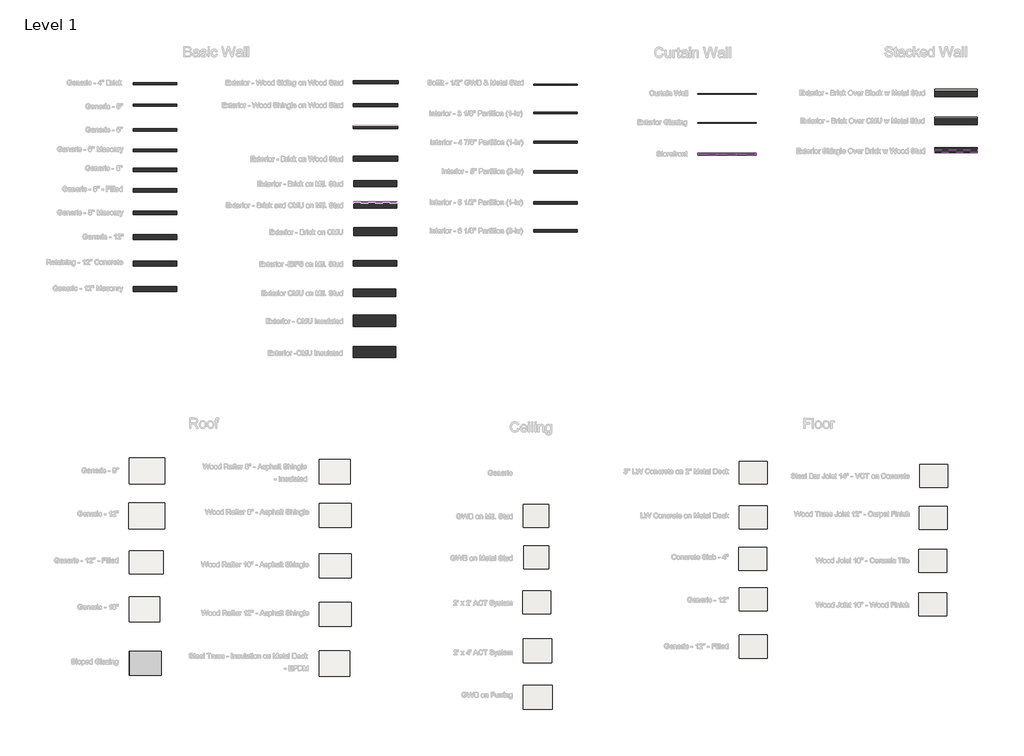
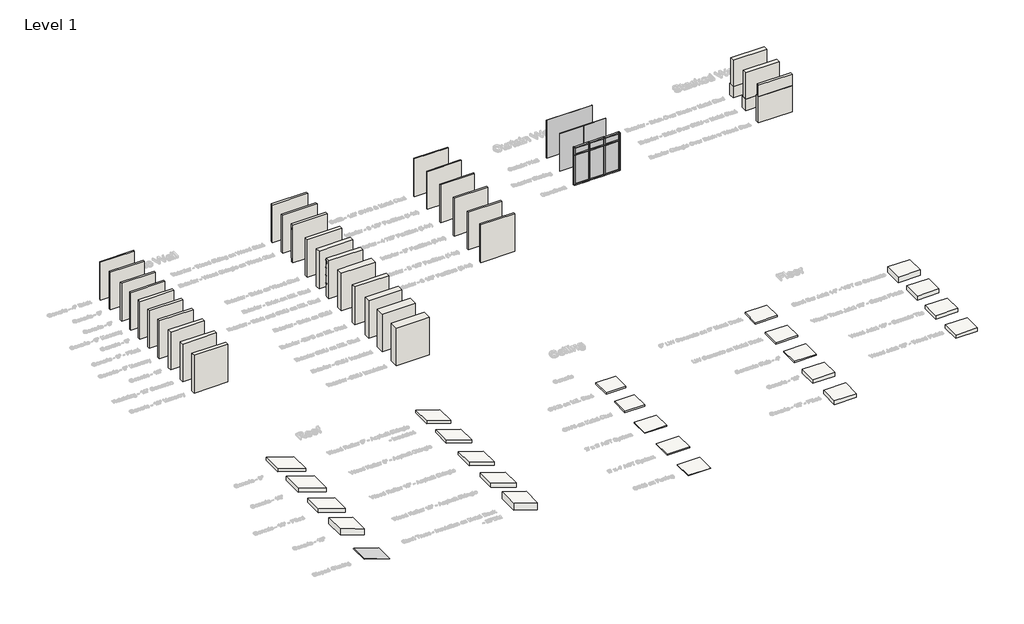
# One storey, part 1 of 42: 33 walls, 17 members, 10 plates, 9 roofs, 9 slabs, 5 coverings, 3 proxies.
# Revit data of these elements (continued)
# Type "Wood Joist 10\" - Wood Finish" (continued)
#   Layers, outside or top first: 0' - 0 3/4" "Oak Flooring" (function 4); 0' - 0 3/4" "Plywood, Sheathing" (function 1); 0' - 9 1/4" "Structure, Wood Joist/Rafter Layer" (function 1)
# Type "Soffit - 1/2\" GWB & Metal Stud"
#   Assembly Code = "B2010"
#   Layers, outside or top first: 0' - 1 1/2" "Metal Furring" (function 1); 0' - 0 1/2" "Gypsum Wall Board" (function 5)
# Type "Exterior - Wood Shingle over Wood Siding on Wood Stud"
#   Assembly Code = "B2010"
#   Layers, outside or top first: 0' - 0 5/8" "Wood Shake" (function 4); 0' - 0 5/8" "Siding, Clapboard" (function 4); 0' - 0" "Air Infiltration Barrier" (function 100); 0' - 0 3/4" "Plywood, Sheathing" (function 2); 0' - 5 1/2" "Softwood, Lumber" (function 1); 0' - 0" "Vapor Retarder" (function 100); 0' - 0 1/2" "Gypsum Wall Board" (function 5)
# Type "Exterior - Block on Mtl. Stud"
#   Layers, outside or top first: 0' - 7.87402" "Concrete Masonry Units" (function 4); 0' - 2.99213" "Air" (function 3); 0' - 0" "Air Infiltration Barrier" (function 100); 0' - 0.74803" "Plywood, Sheathing" (function 2); 0' - 5.98425" "Metal Stud Layer" (function 1); 0' - 0" "Vapour Retarder" (function 100); 0' - 0.51181" "Gypsum Wall Board" (function 5)
# Type "Exterior - Brick and CMU on MTL. Stud"
#   Assembly Code = "B2010"
#   Layers, outside or top first: 0' - 3 5/8" "Brick, Common" (function 4); 0' - 3 5/8" "Concrete Masonry Units" (function 4); 0' - 3" "Air" (function 3); 0' - 0" "Air Infiltration Barrier" (function 100); 0' - 0 3/4" "Plywood, Sheathing" (function 2); 0' - 6" "Metal Stud Layer" (function 1); 0' - 0" "Vapor Retarder" (function 100); 0' - 0 1/2" "Gypsum Wall Board" (function 5)
# Type "Exterior - Brick on CMU"
#   Assembly Code = "B2010156"
#   Layers, outside or top first: 0' - 3 5/8" "Brick, Common" (function 4); 0' - 3" "Air" (function 3); 0' - 3" "Rigid insulation" (function 3); 0' - 0" "Damp-proofing" (function 100); 0' - 7 5/8" "Concrete Masonry Units" (function 1); 0' - 1 5/8" "Metal Furring" (function 2); 0' - 0 5/8" "Gypsum Wall Board" (function 5)
# Type "Exterior - Brick on Mtl. Stud"
#   Assembly Code = "B2010158"
#   Layers, outside or top first: 0' - 3 5/8" "Brick, Common" (function 4); 0' - 3" "Air" (function 3); 0' - 0" "Air Infiltration Barrier" (function 100); 0' - 0 3/4" "Plywood, Sheathing" (function 2); 0' - 6" "Metal Stud Layer" (function 1); 0' - 0" "Vapor Retarder" (function 100); 0' - 0 1/2" "Gypsum Wall Board" (function 5)
# Type "Exterior - Brick on Wood Stud"
#   Assembly Code = "B2010158"
#   Layers, outside or top first: 0' - 3 5/8" "Brick, Common" (function 4); 0' - 1" "Air" (function 3); 0' - 0" "Air Infiltration Barrier" (function 100); 0' - 0 1/2" "Plywood, Sheathing" (function 2); 0' - 5 1/2" "Softwood, Lumber" (function 1); 0' - 0" "Vapor Retarder" (function 100); 0' - 0 1/2" "Gypsum Wall Board" (function 5)
# Type "Exterior - CMU Insulated"
#   Assembly Code = "B2010144"
#   Layers, outside or top first: 0' - 7 5/8" "Concrete Masonry Units" (function 1); 0' - 2" "Air" (function 3); 0' - 3" "Rigid insulation" (function 3); 0' - 0" "Damp-proofing" (function 100); 0' - 11 5/8" "Concrete Masonry Units" (function 1); 0' - 1 5/8" "Metal Furring" (function 2); 0' - 0 5/8" "Gypsum Wall Board" (function 5)
# Type "Exterior - CMU on Mtl. Stud"
#   Assembly Code = "B2010158"
#   Layers, outside or top first: 0' - 7 5/8" "Concrete Masonry Units" (function 4); 0' - 3" "Air" (function 3); 0' - 0" "Air Infiltration Barrier" (function 100); 0' - 0 3/4" "Plywood, Sheathing" (function 2); 0' - 6" "Metal Stud Layer" (function 1); 0' - 0" "Vapor Retarder" (function 100); 0' - 0 1/2" "Gypsum Wall Board" (function 5)
# Type "Exterior - EIFS on Mtl. Stud"
#   Assembly Code = "B2010100"
#   Layers, outside or top first: 0' - 3" "EIFS, Exterior Insulation" (function 4); 0' - 2" "Air" (function 3); 0' - 0" "Air Infiltration Barrier" (function 100); 0' - 0 3/4" "Plywood, Sheathing" (function 2); 0' - 6" "Metal Stud Layer" (function 1); 0' - 0" "Vapor Retarder" (function 100); 0' - 0 1/2" "Gypsum Wall Board" (function 5)
# Type "Exterior - Wood Shingle on Wood Stud"
#   Assembly Code = "B2010100"
#   Layers, outside or top first: 0' - 0 5/8" "Wood Shake" (function 4); 0' - 0" "Air Infiltration Barrier" (function 100); 0' - 0 1/2" "Plywood, Sheathing" (function 2); 0' - 5 1/2" "Softwood, Lumber" (function 1); 0' - 0" "Vapor Retarder" (function 100); 0' - 0 1/2" "Gypsum Wall Board" (function 5)
# Type "Exterior - Wood Siding on Wood Stud"
#   Assembly Code = "B2010100"
#   Layers, outside or top first: 0' - 0 3/4" "Siding, Clapboard" (function 4); 0' - 0" "Air Infiltration Barrier" (function 100); 0' - 0 1/2" "Plywood, Sheathing" (function 2); 0' - 5 1/2" "Softwood, Lumber" (function 1); 0' - 0" "Vapor Retarder" (function 100); 0' - 0 1/2" "Gypsum Wall Board" (function 5)
# Type "Generic - 12\""
#   Assembly Code = "B2010"
#   Layers, outside or top first: 1' - 0" no material (function 1)
# Type "Generic - 12\" Masonry"
#   Assembly Code = "B2010"
#   Layers, outside or top first: 0' - 11 5/8" "Concrete Masonry Units" (function 1)
# Type "Generic - 4\" Brick"
#   Assembly Code = "B2010"
#   Layers, outside or top first: 0' - 4" "Brick, Common" (function 1)
# Type "Generic - 5\""
#   Assembly Code = "B2010"
#   Layers, outside or top first: 0' - 5" no material (function 1)
# Type "Generic - 6\""
#   Assembly Code = "B2010"
#   Layers, outside or top first: 0' - 6" no material (function 1)
# Type "Generic - 6\" Masonry"
#   Assembly Code = "B2010"
#   Layers, outside or top first: 0' - 5 5/8" "Concrete Masonry Units" (function 1)
# Type "Generic - 8\""
#   Assembly Code = "B2010"
#   Layers, outside or top first: 0' - 8" no material (function 1)
# Type "Generic - 8\" - Filled"
#   Assembly Code = "B2010"
#   Layers, outside or top first: 0' - 8" no material (function 1)
# Type "Generic - 8\" Masonry"
#   Assembly Code = "B2010"
#   Layers, outside or top first: 0' - 7 5/8" "Concrete Masonry Units" (function 1)
# Type "Interior - 3 1/8\" Partition (1-hr)"
#   Assembly Code = "C1010145"
#   Layers, outside or top first: 0' - 0 1/2" "Gypsum Wall Board" (function 5); 0' - 0 1/4" "Gypsum Wall Board" (function 5); 0' - 1 5/8" "Metal Stud Layer" (function 1); 0' - 0 1/4" "Gypsum Wall Board" (function 5); 0' - 0 1/2" "Gypsum Wall Board" (function 5)
# Type "Interior - 4 7/8\" Partition (1-hr)"
#   Assembly Code = "C1010145"
#   Layers, outside or top first: 0' - 0 5/8" "Gypsum Wall Board" (function 5); 0' - 3 5/8" "Metal Stud Layer" (function 1); 0' - 0 5/8" "Gypsum Wall Board" (function 5)
# Type "Interior - 5 1/2\" Partition (1-hr)"
#   Assembly Code = "C1010145"
#   Layers, outside or top first: 0' - 0 5/8" "Gypsum Wall Board" (function 5); 0' - 3 5/8" "Metal Stud Layer" (function 1); 0' - 0 5/8" "Gypsum Wall Board" (function 5); 0' - 0 5/8" "Gypsum Wall Board" (function 5)
# Type "Interior - 5\" Partition (2-hr)"
#   Assembly Code = "C1010145"
#   Layers, outside or top first: 0' - 0 5/8" "Gypsum Wall Board" (function 5); 0' - 0 5/8" "Gypsum Wall Board" (function 5); 0' - 2 1/2" "Metal Stud Layer" (function 1); 0' - 0 5/8" "Gypsum Wall Board" (function 5); 0' - 0 5/8" "Gypsum Wall Board" (function 5)
# Type "Interior - 6 1/8\" Partition (2-hr)"
#   Assembly Code = "C1010145"
#   Layers, outside or top first: 0' - 0 5/8" "Gypsum Wall Board" (function 5); 0' - 0 5/8" "Gypsum Wall Board" (function 5); 0' - 3 5/8" "Metal Stud Layer" (function 1); 0' - 0 5/8" "Gypsum Wall Board" (function 5); 0' - 0 5/8" "Gypsum Wall Board" (function 5)
# Type "Retaining - 12\" Concrete"
#   Layers, outside or top first: 1' - 0" "Concrete, Cast-in-Place gray" (function 1)
# Element 4 (IfcCovering, "2' x 2' ACT System")
#   Height Offset From Level = 1' - 0"
#   Phase Created = New Construction
#   Materials on its faces: "Acoustic Ceiling Tile 24 x 24", "Default"
# Element 5 (IfcCovering, "2' x 4' ACT System")
#   Height Offset From Level = 1' - 0"
#   Phase Created = New Construction
#   Materials on its faces: "Acoustic Ceiling Tile 24 x 48", "Default"
# Element 6 (IfcCovering, "GWB on Furring")
#   Height Offset From Level = 1' - 0"
#   Phase Created = New Construction
#   Materials on its faces: "Gypsum Wall Board", "Metal Stud Layer"
# Element 7 (IfcCovering, "GWB on Metal Stud")
#   Height Offset From Level = 1' - 0"
#   Phase Created = New Construction
#   Materials on its faces: "Gypsum Wall Board", "Metal Stud Layer"
# Element 8 (IfcCovering, "GWB on Mtl. Stud")
#   Height Offset From Level = 1' - 0"
#   Phase Created = New Construction
#   Materials on its faces: "Gypsum Wall Board", "Metal Stud Layer"
# Elements 9, 10, 11, 12, 13, 14, 15, 16, 17, 18, 19, 20, 21, 22, 23, 24, 25 (IfcMember, "Rectangular Mullion : 2.5\" x 5\" rectangular")
#   Phase Created = New Construction
#   Materials on its faces: "Aluminum"
# Elements 26, 27, 28, 29, 30, 31, 32, 33, 34, 35 (IfcPlate, "System Panel : Glazed")
#   Phase Created = New Construction
#   Materials on its faces: "Glass"
# Element 36 (IfcRoof, "Generic - 12\"")
#   built-in parameter 1001705 = 3.40154 (stored number, unit not read)
#   built-in parameter 1001710 = 33615
#   Phase Created = New Construction
#   Materials on its faces: "Default Roof"
# Element 37 (IfcRoof, "Generic - 12\" - Filled")
#   built-in parameter 1001705 = 3.29103 (stored number, unit not read)
#   built-in parameter 1001710 = 33615
#   Phase Created = New Construction
#   Materials on its faces: "Default Roof"
# Element 38 (IfcRoof, "Generic - 18\"")
#   built-in parameter 1001705 = 3.60503 (stored number, unit not read)
#   built-in parameter 1001710 = 33615
#   Phase Created = New Construction
#   Materials on its faces: "Default Roof"
# Element 39 (IfcRoof, "Generic - 9\"")
#   built-in parameter 1001705 = 3.1239 (stored number, unit not read)
#   built-in parameter 1001710 = 33615
#   Phase Created = New Construction
#   Materials on its faces: "Default Roof"
# Element 40 (IfcRoof, "Steel Truss - Insulation on Metal Deck - EPDM")
#   built-in parameter 1001705 = 3.88858 (stored number, unit not read)
#   built-in parameter 1001710 = 33615
#   Phase Created = New Construction
#   Materials on its faces: "Structure, Steel Bar Joist Layer", "Roofing, EPDM Membrane"
# Element 41 (IfcRoof, "Wood Rafter 10\" - Asphalt Shingle")
#   built-in parameter 1001705 = 3.00948 (stored number, unit not read)
#   built-in parameter 1001710 = 33615
#   Phase Created = New Construction
#   Materials on its faces: "Structure, Wood Joist/Rafter Layer, Batt Insulation", "Asphalt Shingle"
# Element 42 (IfcRoof, "Wood Rafter 12\" - Asphalt Shingle")
#   built-in parameter 1001705 = 3.18516 (stored number, unit not read)
#   built-in parameter 1001710 = 33615
#   Phase Created = New Construction
#   Materials on its faces: "Structure, Wood Joist/Rafter Layer, Batt Insulation", "Asphalt Shingle"
# Element 43 (IfcRoof, "Wood Rafter 8\" - Asphalt Shingle")
#   built-in parameter 1001705 = 2.8338 (stored number, unit not read)
#   built-in parameter 1001710 = 33615
#   Phase Created = New Construction
#   Materials on its faces: "Structure, Wood Joist/Rafter Layer, Batt Insulation", "Asphalt Shingle"
# Element 44 (IfcRoof, "Wood Rafter 8\" - Asphalt Shingle - Insulated")
#   built-in parameter 1001705 = 2.75956 (stored number, unit not read)
#   built-in parameter 1001710 = 33615
#   Phase Created = New Construction
#   Materials on its faces: "Structure, Wood Joist/Rafter Layer, Batt Insulation", "Asphalt Shingle"
# Element 45 (IfcSlab, "Wood Truss  Joist 12\" - Carpet Finish ")
#   Height Offset From Level = 0' - 0"
#   Phase Created = New Construction
#   Materials on its faces: "Structure, Wood Joist/Rafter Layer", "Carpet (1)"
# Element 46 (IfcSlab, "3\" LW Concrete on 2\" Metal Deck")
#   Height Offset From Level = 0' - 0"
#   Phase Created = New Construction
#   Materials on its faces: "Metal Deck", "Concrete, Lightweight"
# Element 47 (IfcSlab, "Concrete Slab - 4\"")
#   Height Offset From Level = 0' - 0"
#   Phase Created = New Construction
#   Materials on its faces: "Concrete, Cast-in-Place gray"
# Element 48 (IfcSlab, "Generic - 12\"")
#   Height Offset From Level = 0' - 0"
#   Phase Created = New Construction
#   Materials on its faces: "Default Floor"
# Element 49 (IfcSlab, "Generic - 12\" - Filled")
#   Height Offset From Level = 0' - 0"
#   Phase Created = New Construction
#   Materials on its faces: "Default Floor"
# Element 50 (IfcSlab, "LW Concrete on Metal Deck")
#   Height Offset From Level = 0' - 0"
#   Phase Created = New Construction
#   Materials on its faces: "Metal Deck", "Concrete, Lightweight"
# Element 51 (IfcSlab, "Steel Bar Joist 14\" - VCT on Concrete")
#   Height Offset From Level = 0' - 0"
#   Phase Created = New Construction
#   Materials on its faces: "Structure, Steel Bar Joist Layer", "Vinyl Composition Tile"
# Element 52 (IfcSlab, "Wood Joist 10\" - Ceramic Tile")
#   Height Offset From Level = 0' - 0"
#   Phase Created = New Construction
#   Materials on its faces: "Structure, Wood Joist/Rafter Layer", "Tile, Mosaic, Gray"
# Element 53 (IfcSlab, "Wood Joist 10\" - Wood Finish")
#   Height Offset From Level = 0' - 0"
#   Phase Created = New Construction
#   Materials on its faces: "Structure, Wood Joist/Rafter Layer", "Oak Flooring"
# Element 54 (IfcWall, "Soffit - 1/2\" GWB & Metal Stud")
#   Top Offset = 0' - 0"
#   Base Offset = 0' - 0"
#   Unconnected Height = 10' - 0"
#   wall height = 10' - 0"
#   Phase Created = New Construction
#   Base Constraint = Level 1
#   Materials on its faces: "Default Wall", "Gypsum Wall Board", "Metal Furring"
# Element 55 (IfcWall, "Exterior - Wood Shingle over Wood Siding on Wood Stud")
#   Top Offset = 0' - 0"
#   Base Offset = 0' - 0"
#   Unconnected Height = 10' - 0"
#   wall height = 10' - 0"
#   Phase Created = New Construction
#   Base Constraint = Level 1
#   Materials on its faces: "Default Wall", "Gypsum Wall Board", "Siding, Clapboard"
# Element 56 (IfcWall, "Exterior - Block on Mtl. Stud")
#   Top Offset = 0' - 0"
#   Base Offset = 0' - 0"
#   Unconnected Height = 2' - 11.43307"
#   wall height = 2' - 11.43307"
#   Phase Created = New Construction
#   Base Constraint = Level 1
#   Materials on its faces: "Default Wall", "Gypsum Wall Board", "Concrete Masonry Units"
# Element 57 (IfcWall, "Exterior - Brick and CMU on MTL. Stud")
#   Top Offset = 0' - 0"
#   Base Offset = 0' - 0"
#   Unconnected Height = 10' - 0"
#   wall height = 10' - 0"
#   Phase Created = New Construction
#   Base Constraint = Level 1
#   Materials on its faces: "Brick, Common", "Default Wall", "Concrete Masonry Units", "Gypsum Wall Board"
# Element 58 (IfcWall, "Exterior - Brick on CMU")
#   Top Offset = 0' - 0"
#   Base Offset = 0' - 0"
#   Unconnected Height = 10' - 0"
#   wall height = 10' - 0"
#   Phase Created = New Construction
#   Base Constraint = Level 1
#   Materials on its faces: "Default Wall", "Gypsum Wall Board", "Brick, Common"
# Element 59 (IfcWall, "Exterior - Brick on Mtl. Stud")
#   Top Offset = 0' - 0"
#   Base Offset = 0' - 0"
#   Unconnected Height = 10' - 0"
#   wall height = 10' - 0"
#   Phase Created = New Construction
#   Base Constraint = Level 1
#   Materials on its faces: "Default Wall", "Gypsum Wall Board", "Brick, Common"
# Element 60 (IfcWall, "Exterior - Brick on Mtl. Stud")
#   built-in parameter 1001111 = 2' - 11.43307"
#   Top Offset = 0' - 0"
#   Base Offset = 2' - 11.43307"
#   Unconnected Height = 7' - 0.56693"
#   wall height = 7' - 0.56693"
#   Phase Created = New Construction
#   Base Constraint = Level 1
#   Materials on its faces: "Default Wall", "Gypsum Wall Board", "Brick, Common"
# Element 61 (IfcWall, "Exterior - Brick on Mtl. Stud")
#   built-in parameter 1001111 = 3' - 0"
#   Top Offset = 0' - 0"
#   Base Offset = 3' - 0"
#   Unconnected Height = 7' - 0"
#   wall height = 7' - 0"
#   Phase Created = New Construction
#   Base Constraint = Level 1
#   Materials on its faces: "Default Wall", "Gypsum Wall Board", "Brick, Common"
# Element 62 (IfcWall, "Exterior - Brick on Wood Stud")
#   Top Offset = 0' - 0"
#   Base Offset = 0' - 0"
#   Unconnected Height = 10' - 0"
#   wall height = 10' - 0"
#   Phase Created = New Construction
#   Base Constraint = Level 1
#   Materials on its faces: "Default Wall", "Gypsum Wall Board", "Brick, Common"
# Element 63 (IfcWall, "Exterior - Brick on Wood Stud")
#   Top Offset = 0' - 0"
#   Base Offset = 0' - 0"
#   Unconnected Height = 7' - 0"
#   wall height = 7' - 0"
#   Phase Created = New Construction
#   Base Constraint = Level 1
#   Materials on its faces: "Default Wall", "Gypsum Wall Board", "Brick, Common"
# Elements 64, 65 (IfcWall, "Exterior - CMU Insulated")
#   Top Offset = 0' - 0"
#   Base Offset = 0' - 0"
#   Unconnected Height = 10' - 0"
#   wall height = 10' - 0"
#   Phase Created = New Construction
#   Base Constraint = Level 1
#   Materials on its faces: "Default Wall", "Gypsum Wall Board", "Concrete Masonry Units"
# Element 66 (IfcWall, "Exterior - CMU on Mtl. Stud")
#   Top Offset = 0' - 0"
#   Base Offset = 0' - 0"
#   Unconnected Height = 10' - 0"
#   wall height = 10' - 0"
#   Phase Created = New Construction
#   Base Constraint = Level 1
#   Materials on its faces: "Default Wall", "Gypsum Wall Board", "Concrete Masonry Units"
# Element 67 (IfcWall, "Exterior - CMU on Mtl. Stud")
#   Top Offset = 0' - 0"
#   Base Offset = 0' - 0"
#   Unconnected Height = 3' - 0"
#   wall height = 3' - 0"
#   Phase Created = New Construction
#   Base Constraint = Level 1
#   Materials on its faces: "Default Wall", "Gypsum Wall Board", "Concrete Masonry Units"
# Element 68 (IfcWall, "Exterior - EIFS on Mtl. Stud")
#   Top Offset = 0' - 0"
#   Base Offset = 0' - 0"
#   Unconnected Height = 10' - 0"
#   wall height = 10' - 0"
#   Phase Created = New Construction
#   Base Constraint = Level 1
#   Materials on its faces: "Default Wall", "Gypsum Wall Board", "EIFS, Exterior Insulation"
# Element 69 (IfcWall, "Exterior - Wood Shingle on Wood Stud")
#   Top Offset = 0' - 0"
#   Base Offset = 0' - 0"
#   Unconnected Height = 10' - 0"
#   wall height = 10' - 0"
#   Phase Created = New Construction
#   Base Constraint = Level 1
#   Materials on its faces: "Default Wall", "Gypsum Wall Board", "Wood Shake"
# Element 70 (IfcWall, "Exterior - Wood Shingle on Wood Stud")
#   built-in parameter 1001111 = 7' - 0"
#   Top Offset = 0' - 0"
#   Base Offset = 7' - 0"
#   Unconnected Height = 3' - 0"
#   wall height = 3' - 0"
#   Phase Created = New Construction
#   Base Constraint = Level 1
#   Materials on its faces: "Default Wall", "Gypsum Wall Board", "Wood Shake"
# Element 71 (IfcWall, "Exterior - Wood Siding on Wood Stud")
#   Top Offset = 0' - 0"
#   Base Offset = 0' - 0"
#   Unconnected Height = 10' - 0"
#   wall height = 10' - 0"
#   Phase Created = New Construction
#   Base Constraint = Level 1
#   Materials on its faces: "Default Wall", "Gypsum Wall Board", "Siding, Clapboard"
# Element 72 (IfcWall, "Generic - 12\"")
#   Top Offset = 0' - 0"
#   Base Offset = 0' - 0"
#   Unconnected Height = 10' - 0"
#   wall height = 10' - 0"
#   Phase Created = New Construction
#   Base Constraint = Level 1
#   Materials on its faces: "Default Wall"
# Element 73 (IfcWall, "Generic - 12\" Masonry")
#   Top Offset = 0' - 0"
#   Base Offset = 0' - 0"
#   Unconnected Height = 10' - 0"
#   wall height = 10' - 0"
#   Phase Created = New Construction
#   Base Constraint = Level 1
#   Materials on its faces: "Concrete Masonry Units"
# Element 74 (IfcWall, "Generic - 4\" Brick")
#   Top Offset = 0' - 0"
#   Base Offset = 0' - 0"
#   Unconnected Height = 10' - 0"
#   wall height = 10' - 0"
#   Phase Created = New Construction
#   Base Constraint = Level 1
#   Materials on its faces: "Brick, Common"
# Element 75 (IfcWall, "Generic - 5\"")
#   Top Offset = 0' - 0"
#   Base Offset = 0' - 0"
#   Unconnected Height = 10' - 0"
#   wall height = 10' - 0"
#   Phase Created = New Construction
#   Base Constraint = Level 1
#   Materials on its faces: "Default Wall"
# Element 76 (IfcWall, "Generic - 6\"")
#   Top Offset = 0' - 0"
#   Base Offset = 0' - 0"
#   Unconnected Height = 10' - 0"
#   wall height = 10' - 0"
#   Phase Created = New Construction
#   Base Constraint = Level 1
#   Materials on its faces: "Default Wall"
# Element 77 (IfcWall, "Generic - 6\" Masonry")
#   Top Offset = 0' - 0"
#   Base Offset = 0' - 0"
#   Unconnected Height = 10' - 0"
#   wall height = 10' - 0"
#   Phase Created = New Construction
#   Base Constraint = Level 1
#   Materials on its faces: "Concrete Masonry Units"
# Element 78 (IfcWall, "Generic - 8\"")
#   Top Offset = 0' - 0"
#   Base Offset = 0' - 0"
#   Unconnected Height = 10' - 0"
#   wall height = 10' - 0"
#   Phase Created = New Construction
#   Base Constraint = Level 1
#   Materials on its faces: "Default Wall"
# Element 79 (IfcWall, "Generic - 8\" - Filled")
#   Top Offset = 0' - 0"
#   Base Offset = 0' - 0"
#   Unconnected Height = 10' - 0"
#   wall height = 10' - 0"
#   Phase Created = New Construction
#   Base Constraint = Level 1
#   Materials on its faces: "Default Wall"
# Element 80 (IfcWall, "Generic - 8\" Masonry")
#   Top Offset = 0' - 0"
#   Base Offset = 0' - 0"
#   Unconnected Height = 10' - 0"
#   wall height = 10' - 0"
#   Phase Created = New Construction
#   Base Constraint = Level 1
#   Materials on its faces: "Concrete Masonry Units"
# Element 81 (IfcWall, "Interior - 3 1/8\" Partition (1-hr)")
#   Top Offset = 0' - 0"
#   Base Offset = 0' - 0"
#   wall height = 10' - 0"
#   Phase Created = New Construction
#   Base Constraint = Level 1
#   Top Constraint = Level 2
#   Materials on its faces: "Default Wall", "Gypsum Wall Board"
# Element 82 (IfcWall, "Interior - 4 7/8\" Partition (1-hr)")
#   Top Offset = 0' - 0"
#   Base Offset = 0' - 0"
#   wall height = 10' - 0"
#   Phase Created = New Construction
#   Base Constraint = Level 1
#   Top Constraint = Level 2
#   Materials on its faces: "Default Wall", "Gypsum Wall Board"
# Element 83 (IfcWall, "Interior - 5 1/2\" Partition (1-hr)")
#   Top Offset = 0' - 0"
#   Base Offset = 0' - 0"
#   wall height = 10' - 0"
#   Phase Created = New Construction
#   Base Constraint = Level 1
#   Top Constraint = Level 2
#   Materials on its faces: "Default Wall", "Gypsum Wall Board"
# Element 84 (IfcWall, "Interior - 5\" Partition (2-hr)")
#   Top Offset = 0' - 0"
#   Base Offset = 0' - 0"
#   wall height = 10' - 0"
#   Phase Created = New Construction
#   Base Constraint = Level 1
#   Top Constraint = Level 2
#   Materials on its faces: "Default Wall", "Gypsum Wall Board"
# Element 85 (IfcWall, "Interior - 6 1/8\" Partition (2-hr)")
#   Top Offset = 0' - 0"
#   Base Offset = 0' - 0"
#   wall height = 10' - 0"
#   Phase Created = New Construction
#   Base Constraint = Level 1
#   Top Constraint = Level 2
#   Materials on its faces: "Default Wall", "Gypsum Wall Board"
# Element 86 (IfcWall, "Retaining - 12\" Concrete")
#   Top Offset = 0' - 0"
#   Base Offset = 0' - 0"
#   Unconnected Height = 10' - 0"
#   wall height = 10' - 0"
#   Phase Created = New Construction
#   Base Constraint = Level 1
#   Materials on its faces: "Concrete, Cast-in-Place gray"
# Materials
#   "Default": class "Miscellaneous", colour RGB 127 127 127, transparency 0, Cost = 0
#   "Acoustic Ceiling Tile 24 x 24": class "Generic", colour RGB 232 232 232, transparency 0, Description = "Acoustic Ceiling Tile 24 x 24", Cost = 0
#   "Acoustic Ceiling Tile 24 x 48": class "Generic", colour RGB 229 229 229, transparency 0, Description = "Acoustic Ceiling Tile 24 x 48", Cost = 0
#   "Metal Stud Layer": class "Metal", colour RGB 199 199 199, transparency 0, Description = "Light gauge steel framing, thermal air layer", Cost = 0
#   "Gypsum Wall Board": class "Generic", colour RGB 127 127 127, transparency 0, Description = "Gypsum Wall Board", Cost = 0
#   "Roofing, EPDM Membrane": class "Generic", colour RGB 127 127 127, transparency 0, Description = "EPDM roof membrane", Cost = 0
#   "Rigid insulation": class "Generic", colour RGB 127 127 127, transparency 0, Description = "Rigid foam insulation board", Cost = 0
#   "Metal Deck": class "Metal", colour RGB 199 199 199, transparency 0, Description = "Steel, mill finish", Cost = 0
#   "Structure, Steel Bar Joist Layer": class "Metal", colour RGB 127 127 127, transparency 0, Description = "Bar joists, thermal airspace", Cost = 0
#   "Asphalt Shingle": class "Generic", colour RGB 155 155 155, transparency 0, Description = "Asphalt roofing shingle", Cost = 0
#   "Plywood, Sheathing": class "Wood", colour RGB 212 179 113, transparency 0, Description = "Plywood, sheathing grade", Cost = 0
#   "Structure, Wood Joist/Rafter Layer, Batt Insulation": class "Wood", colour RGB 127 127 127, transparency 0, Description = "Wood framing, insulated", Cost = 0
#   "Carpet (1)": class "Carpet", colour RGB 124 80 67, transparency 0, Description = "Interior finish", Cost = 0
#   "Structure, Wood Joist/Rafter Layer": class "Wood", colour RGB 127 127 127, transparency 0, Description = "Wood framing, thermal airspace", Cost = 0
#   "Concrete, Lightweight": class "Concrete", colour RGB 142 141 140, transparency 0, Description = "Lightweight concrete", Cost = 0
#   "Concrete, Cast-in-Place gray": class "Concrete", colour RGB 192 192 192, transparency 0, Description = "Cast-in-place concrete", Cost = 0
#   "Vinyl Composition Tile": class "Generic", colour RGB 179 160 124, transparency 0, Description = "Vinyl Composition Tile", Cost = 0
#   "Tile, Mosaic, Gray": class "Generic", colour RGB 127 127 127, transparency 0, Description = "Mosiac tile, gray", Cost = 0
#   "Oak Flooring": class "Wood", colour RGB 216 169 114, transparency 0, Description = "Quercus Rubra", Cost = 0
#   "Metal Furring": class "Metal", colour RGB 199 199 199, transparency 0, Description = "Light gauge steel furring", Cost = 0
#   "Wood Shake": class "Wood", colour RGB 151 131 103, transparency 0, Description = "Wood roofing shakes", Cost = 0
#   "Siding, Clapboard": class "Wood", colour RGB 242 231 197, transparency 0, Description = "Softwood clapboard siding", Cost = 0
#   "Air Infiltration Barrier": class "Generic", colour RGB 127 127 127, transparency 0, Description = "physical material", Cost = 0
#   "Softwood, Lumber": class "Wood", colour RGB 223 192 134, transparency 0, Description = "Pinus Echinata", Cost = 0
#   "Vapor Retarder": class "Generic", colour RGB 127 127 127, transparency 0, Description = "Polyethylene film membrane", Cost = 0
#   "Concrete Masonry Units": class "Masonry", colour RGB 227 227 227, transparency 0, Description = "Concrete masonry units", Cost = 0
#   "Air": class "Gas", colour RGB 255 255 255, transparency 0, Description = "Air", Cost = 0
#   "Vapour Retarder": class "Generic", colour RGB 127 127 127, transparency 0, Description = "Polyethylene film membrane", Cost = 0
#   "Brick, Common": class "Masonry", colour RGB 170 98 104, transparency 0, Description = "Common brick", Cost = 0
#   "Damp-proofing": class "Generic", colour RGB 127 127 127, transparency 0, Description = "Damp-proofing", Cost = 0
#   "EIFS, Exterior Insulation": class "Generic", colour RGB 127 127 127, transparency 0, Description = "EIFS - Exterior Insulation", Cost = 0
#   "Aluminum": class "Metal", colour RGB 247 247 247, transparency 0, Description = "Aluminum 6061", Cost = 0
#   "Glass": class "Glass", colour RGB 0 128 192, transparency 0.75, Description = "Soda Lime Glass", Cost = 0
#   "Default Roof": class "Miscellaneous", colour RGB 88 101 114, transparency 0, Cost = 0
#   "Default Floor": class "Miscellaneous", colour RGB 128 128 128, transparency 0, Cost = 0
#   "Default Wall": class "Miscellaneous", colour RGB 128 128 128, transparency 0, Cost = 0
